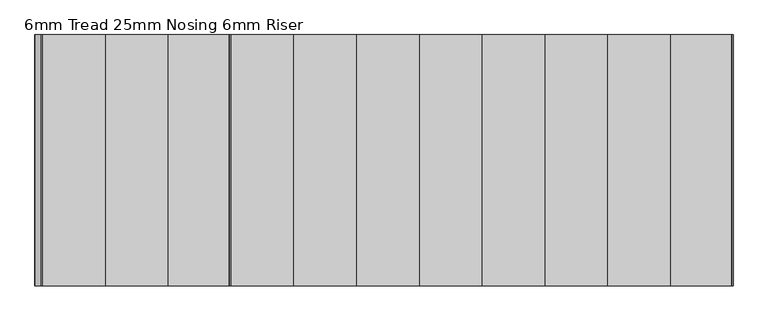
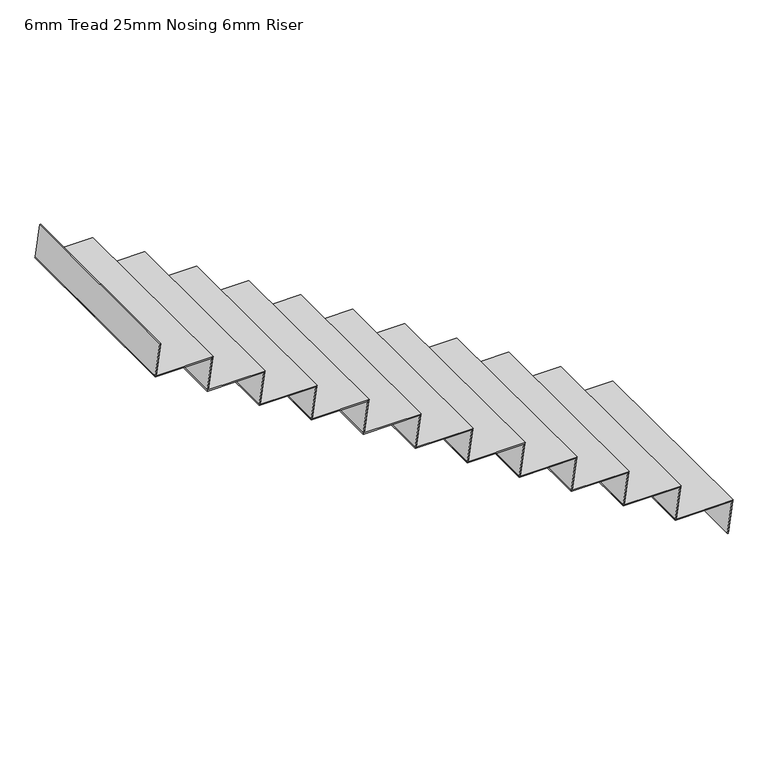
"""IFC4 building model written with IfcOpenShell, lengths in millimetres: stair flight geometry, 6mm Tread 25mm Nosing 6mm Riser."""

from ifc_helpers import new_model, si_unit, frame, origin, place, context, project, spatial, polyline, outline, extrude, source, transform, mapped, element, save


def stair_flight_6mm_tread_25mm_nosing_6mm_riser_34bf7372(model_context):
    return source(origin(), model_context, "Body", "SweptSolid", [
        extrude(outline(polyline([(10117.6470588, 16350.0), (10117.6470588, 16043.9400908), (10111.6470588, 16043.0900908), (10111.6470588, 16349.15), (10117.6470588, 16350.0)])), frame((0.0, 12030.4345331, 0.0), z_axis=(0.0, 1.0, 0.0), x_axis=(0.0, 0.0, 1.0)), (0.0, 0.0, 1.0), 1100.0),
        extrude(outline(polyline([(10111.6470588, 16349.15), (10111.6470588, 16343.0900908), (9941.1764706, 16318.9400908), (9941.1764706, 16325.0), (10111.6470588, 16349.15)])), frame((0.0, 12030.4345331, 0.0), z_axis=(0.0, 1.0, 0.0), x_axis=(0.0, 0.0, 1.0)), (0.0, 0.0, 1.0), 1100.0),
        extrude(outline(polyline([(10288.1176471, 16074.15), (10288.1176471, 16068.0900908), (10117.6470588, 16043.9400908), (10117.6470588, 16050.0), (10288.1176471, 16074.15)])), frame((0.0, 12030.4345331, 0.0), z_axis=(0.0, 1.0, 0.0), x_axis=(0.0, 0.0, 1.0)), (0.0, 0.0, 1.0), 1100.0),
        extrude(outline(polyline([(10294.1176471, 16075.0), (10294.1176471, 15768.9400908), (10288.1176471, 15768.0900908), (10288.1176471, 16074.15), (10294.1176471, 16075.0)])), frame((0.0, 12030.4345331, 0.0), z_axis=(0.0, 1.0, 0.0), x_axis=(0.0, 0.0, 1.0)), (0.0, 0.0, 1.0), 1100.0),
        extrude(outline(polyline([(10464.5882353, 15799.15), (10464.5882353, 15793.0900908), (10294.1176471, 15768.9400908), (10294.1176471, 15775.0), (10464.5882353, 15799.15)])), frame((0.0, 12030.4345331, 0.0), z_axis=(0.0, 1.0, 0.0), x_axis=(0.0, 0.0, 1.0)), (0.0, 0.0, 1.0), 1100.0),
        extrude(outline(polyline([(10470.5882353, 15800.0), (10470.5882353, 15493.9400908), (10464.5882353, 15493.0900908), (10464.5882353, 15799.15), (10470.5882353, 15800.0)])), frame((0.0, 12030.4345331, 0.0), z_axis=(0.0, 1.0, 0.0), x_axis=(0.0, 0.0, 1.0)), (0.0, 0.0, 1.0), 1100.0),
        extrude(outline(polyline([(10641.0588235, 15524.15), (10641.0588235, 15518.0900908), (10470.5882353, 15493.9400908), (10470.5882353, 15500.0), (10641.0588235, 15524.15)])), frame((0.0, 12030.4345331, 0.0), z_axis=(0.0, 1.0, 0.0), x_axis=(0.0, 0.0, 1.0)), (0.0, 0.0, 1.0), 1100.0),
        extrude(outline(polyline([(10647.0588235, 15525.0), (10647.0588235, 15218.9400908), (10641.0588235, 15218.0900908), (10641.0588235, 15524.15), (10647.0588235, 15525.0)])), frame((0.0, 12030.4345331, 0.0), z_axis=(0.0, 1.0, 0.0), x_axis=(0.0, 0.0, 1.0)), (0.0, 0.0, 1.0), 1100.0),
        extrude(outline(polyline([(10817.5294118, 15249.15), (10817.5294118, 15243.0900908), (10647.0588235, 15218.9400908), (10647.0588235, 15225.0), (10817.5294118, 15249.15)])), frame((0.0, 12030.4345331, 0.0), z_axis=(0.0, 1.0, 0.0), x_axis=(0.0, 0.0, 1.0)), (0.0, 0.0, 1.0), 1100.0),
        extrude(outline(polyline([(10823.5294118, 15250.0), (10823.5294118, 14943.9400908), (10817.5294118, 14943.0900908), (10817.5294118, 15249.15), (10823.5294118, 15250.0)])), frame((0.0, 12030.4345331, 0.0), z_axis=(0.0, 1.0, 0.0), x_axis=(0.0, 0.0, 1.0)), (0.0, 0.0, 1.0), 1100.0),
        extrude(outline(polyline([(10994.0, 14974.15), (10994.0, 14968.0900908), (10823.5294118, 14943.9400908), (10823.5294118, 14950.0), (10994.0, 14974.15)])), frame((0.0, 12030.4345331, 0.0), z_axis=(0.0, 1.0, 0.0), x_axis=(0.0, 0.0, 1.0)), (0.0, 0.0, 1.0), 1100.0),
        extrude(outline(polyline([(11000.0, 14975.0), (11000.0, 14668.9400908), (10994.0, 14668.0900908), (10994.0, 14974.15), (11000.0, 14975.0)])), frame((0.0, 12030.4345331, 0.0), z_axis=(0.0, 1.0, 0.0), x_axis=(0.0, 0.0, 1.0)), (0.0, 0.0, 1.0), 1100.0),
        extrude(outline(polyline([(11170.4705882, 14699.15), (11170.4705882, 14693.0900908), (11000.0, 14668.9400908), (11000.0, 14675.0), (11170.4705882, 14699.15)])), frame((0.0, 12030.4345331, 0.0), z_axis=(0.0, 1.0, 0.0), x_axis=(0.0, 0.0, 1.0)), (0.0, 0.0, 1.0), 1100.0),
        extrude(outline(polyline([(11176.4705882, 14700.0), (11176.4705882, 14393.9400908), (11170.4705882, 14393.0900908), (11170.4705882, 14699.15), (11176.4705882, 14700.0)])), frame((0.0, 12030.4345331, 0.0), z_axis=(0.0, 1.0, 0.0), x_axis=(0.0, 0.0, 1.0)), (0.0, 0.0, 1.0), 1100.0),
        extrude(outline(polyline([(11346.9411765, 14424.15), (11346.9411765, 14418.0900908), (11176.4705882, 14393.9400908), (11176.4705882, 14400.0), (11346.9411765, 14424.15)])), frame((0.0, 12030.4345331, 0.0), z_axis=(0.0, 1.0, 0.0), x_axis=(0.0, 0.0, 1.0)), (0.0, 0.0, 1.0), 1100.0),
        extrude(outline(polyline([(11352.9411765, 14425.0), (11352.9411765, 14118.9400908), (11346.9411765, 14118.0900908), (11346.9411765, 14424.15), (11352.9411765, 14425.0)])), frame((0.0, 12030.4345331, 0.0), z_axis=(0.0, 1.0, 0.0), x_axis=(0.0, 0.0, 1.0)), (0.0, 0.0, 1.0), 1100.0),
        extrude(outline(polyline([(11523.4117647, 14149.15), (11523.4117647, 14143.0900908), (11352.9411765, 14118.9400908), (11352.9411765, 14125.0), (11523.4117647, 14149.15)])), frame((0.0, 12030.4345331, 0.0), z_axis=(0.0, 1.0, 0.0), x_axis=(0.0, 0.0, 1.0)), (0.0, 0.0, 1.0), 1100.0),
        extrude(outline(polyline([(11529.4117647, 14150.0), (11529.4117647, 13843.9400908), (11523.4117647, 13843.0900908), (11523.4117647, 14149.15), (11529.4117647, 14150.0)])), frame((0.0, 12030.4345331, 0.0), z_axis=(0.0, 1.0, 0.0), x_axis=(0.0, 0.0, 1.0)), (0.0, 0.0, 1.0), 1100.0),
        extrude(outline(polyline([(11699.8823529, 13874.15), (11699.8823529, 13868.0900908), (11529.4117647, 13843.9400908), (11529.4117647, 13850.0), (11699.8823529, 13874.15)])), frame((0.0, 12030.4345331, 0.0), z_axis=(0.0, 1.0, 0.0), x_axis=(0.0, 0.0, 1.0)), (0.0, 0.0, 1.0), 1100.0),
        extrude(outline(polyline([(11705.8823529, 13875.0), (11705.8823529, 13568.9400908), (11699.8823529, 13568.0900908), (11699.8823529, 13874.15), (11705.8823529, 13875.0)])), frame((0.0, 12030.4345331, 0.0), z_axis=(0.0, 1.0, 0.0), x_axis=(0.0, 0.0, 1.0)), (0.0, 0.0, 1.0), 1100.0),
        extrude(outline(polyline([(11876.3529412, 13599.15), (11876.3529412, 13593.0900908), (11705.8823529, 13568.9400908), (11705.8823529, 13575.0), (11876.3529412, 13599.15)])), frame((0.0, 12030.4345331, 0.0), z_axis=(0.0, 1.0, 0.0), x_axis=(0.0, 0.0, 1.0)), (0.0, 0.0, 1.0), 1100.0),
        extrude(outline(polyline([(12052.8235294, 13324.15), (12052.8235294, 13318.0900908), (11882.3529412, 13293.9400908), (11882.3529412, 13300.0), (12052.8235294, 13324.15)])), frame((0.0, 12030.4345331, 0.0), z_axis=(0.0, 1.0, 0.0), x_axis=(0.0, 0.0, 1.0)), (0.0, 0.0, 1.0), 1100.0),
        extrude(outline(polyline([(11882.3529412, 13600.0), (11882.3529412, 13293.9400908), (11876.3529412, 13293.0900908), (11876.3529412, 13599.15), (11882.3529412, 13600.0)])), frame((0.0, 12030.4345331, 0.0), z_axis=(0.0, 1.0, 0.0), x_axis=(0.0, 0.0, 1.0)), (0.0, 0.0, 1.0), 1100.0),
    ])


if __name__ == "__main__":
    model = new_model("IFC4")
    model_context = context("Model", 3, world=origin())
    ifc_project = project(units=[si_unit("LENGTHUNIT", "METRE", prefix="MILLI")], contexts=[model_context])
    site = spatial("IfcSite", under=ifc_project)
    building = spatial("IfcBuilding", under=site)
    placement = place(None, origin())
    stair_flight_6mm_tread_25mm_nosing_6mm_riser_shape = stair_flight_6mm_tread_25mm_nosing_6mm_riser_34bf7372(model_context)
    element("IfcStairFlight", 1, ObjectType="6mm Tread 25mm Nosing 6mm Riser", at=placement, inside=building, context=model_context, shape_type="MappedRepresentation", body=[
        mapped(stair_flight_6mm_tread_25mm_nosing_6mm_riser_shape, transform((0.0, 0.0, 0.0), x_axis=(1.0, 0.0, 0.0), y_axis=(0.0, 1.0, 0.0), z_axis=(0.0, 0.0, 1.0))),
    ])
    save(model, "model.ifc")

# Revit data of these elements
# Element 1 (IfcStairFlight, "6mm Tread 25mm Nosing 6mm Riser")
#   Materials on its faces: "Steel, Paint Finish, Dark Gray"
# Materials
#   "Steel, Paint Finish, Dark Gray": class "Metal", colour RGB 89 89 89, transparency 0, Description = "Steel, paint finish, dark gray, glossy", Cost = 0
